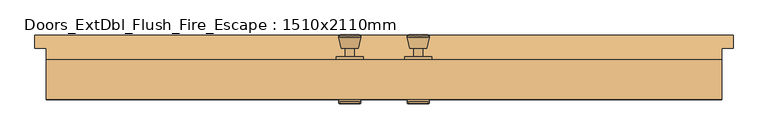
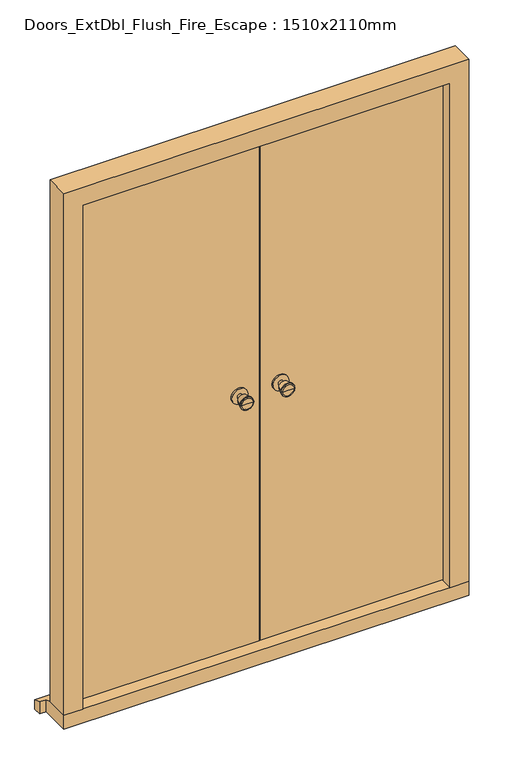
"""IFC4 building model written with IfcOpenShell, lengths in millimetres: door geometry, Doors_ExtDbl_Flush_Fire_Escape : 1510x2110mm."""

import ifcopenshell
import ifcopenshell.guid

model = None  # the IFC model being written
_history = None  # IfcOwnerHistory: only IFC2X3 demands one
_inside = {}  # id of a spatial element -> (the spatial element, [elements in it])
_under = {}  # id of a project, library or spatial element -> (it, [spatial elements below it])
_declared = {}  # id of a project -> (the project, [libraries it declares])
_typed = {}  # id of a type object -> (the type object, [elements of that type])
_made_of = {}  # id of a material, layer set ... -> (it, [elements and type objects made of it])


def new_model(schema):
    """Start an empty IFC model of exactly this schema.

    Asked for "IFC4X3", IfcOpenShell would pick the latest addendum, in which some entities
    have other attributes; the version numbers below select the first issue.
    IFC2X3 requires an IfcOwnerHistory on every rooted entity: one is made here for all.
    """
    global model, _history
    if schema == "IFC4X3":
        model = ifcopenshell.file(schema_version=(4, 3, 0, 0))
    else:
        model = ifcopenshell.file(schema=schema)
    _inside.clear()
    _under.clear()
    _declared.clear()
    _typed.clear()
    _made_of.clear()
    _history = None
    if model.schema == "IFC2X3":
        org = make("IfcOrganization", Name="unknown")
        user = make(
            "IfcPersonAndOrganization",
            ThePerson=make("IfcPerson", FamilyName="unknown"),
            TheOrganization=org,
        )
        app = make(
            "IfcApplication",
            ApplicationDeveloper=org,
            Version="unknown",
            ApplicationFullName="unknown",
            ApplicationIdentifier="unknown",
        )
        _history = make(
            "IfcOwnerHistory",
            OwningUser=user,
            OwningApplication=app,
            ChangeAction="ADDED",
            CreationDate=0,
        )
    return model


def make(cls, **values):
    """One entity of the class cls with the attributes given. An attribute that is None is left unset."""
    return model.create_entity(
        cls, **{name: value for name, value in values.items() if value is not None}
    )


def rooted(cls, **values):
    """An entity with a GlobalId (a new one), such as an element, a storey or a relation."""
    return make(cls, GlobalId=ifcopenshell.guid.new(), OwnerHistory=_history, **values)


def si_unit(unit_type, name, prefix=None):
    """IfcSIUnit, for example si_unit("LENGTHUNIT", "METRE", prefix="MILLI")."""
    return make("IfcSIUnit", UnitType=unit_type, Prefix=prefix, Name=name)


def assignment(units):
    """IfcUnitAssignment: the units of a project."""
    return None if units is None else make("IfcUnitAssignment", Units=units)


def point(xyz):
    """IfcCartesianPoint."""
    return None if xyz is None else make("IfcCartesianPoint", Coordinates=xyz)


def direction(xyz):
    """IfcDirection."""
    return None if xyz is None else make("IfcDirection", DirectionRatios=xyz)


def frame(location, z_axis=None, x_axis=None):
    """IfcAxis2Placement3D, a coordinate frame: its origin and axes. An axis left out is left unset."""
    return make(
        "IfcAxis2Placement3D",
        Location=point(location),
        Axis=direction(z_axis),
        RefDirection=direction(x_axis),
    )


def frame_2d(location, x_axis=None):
    """IfcAxis2Placement2D, a coordinate frame in the plane: its origin and x axis."""
    return make(
        "IfcAxis2Placement2D", Location=point(location), RefDirection=direction(x_axis)
    )


def origin():
    """The frame at (0, 0, 0) with its axes left unset."""
    return frame((0.0, 0.0, 0.0))


def place(relative_to, where):
    """IfcLocalPlacement: puts the frame where relative to a parent placement (None: the world)."""
    return make(
        "IfcLocalPlacement", PlacementRelTo=relative_to, RelativePlacement=where
    )


def context(
    kind, dimensions, precision=None, world=None, true_north=None, identifier=None
):
    """IfcGeometricRepresentationContext, for example the 3D "Model" context."""
    return make(
        "IfcGeometricRepresentationContext",
        ContextIdentifier=identifier,
        ContextType=kind,
        CoordinateSpaceDimension=dimensions,
        Precision=precision,
        WorldCoordinateSystem=world,
        TrueNorth=true_north,
    )


def project(units=None, contexts=None):
    """IfcProject with its units and contexts."""
    return rooted(
        "IfcProject",
        Name="project",
        RepresentationContexts=contexts,
        UnitsInContext=assignment(units),
    )


def spatial(cls, under=None, at=None, **own):
    """A site, building, storey or space (cls), placed at a placement, below another one or the project."""
    s = rooted(cls, ObjectPlacement=at, **own)
    if under is not None:
        _under.setdefault(under.id(), (under, []))[1].append(s)
    return s


def polyline(points):
    """IfcPolyline through the points."""
    return make("IfcPolyline", Points=[point(p) for p in points])


def circle_curve(where, radius):
    """IfcCircle in the frame where."""
    return make("IfcCircle", Position=where, Radius=radius)


def trimmed(basis, trim1, trim2, sense, master):
    """IfcTrimmedCurve: the piece of a basis curve between two trims."""
    return make(
        "IfcTrimmedCurve",
        BasisCurve=basis,
        Trim1=trim1,
        Trim2=trim2,
        SenseAgreement=sense,
        MasterRepresentation=master,
    )


def segment(curve, same_sense, transition):
    """IfcCompositeCurveSegment."""
    return make(
        "IfcCompositeCurveSegment",
        Transition=transition,
        SameSense=same_sense,
        ParentCurve=curve,
    )


def composite_curve(segments, self_intersect=None):
    """IfcCompositeCurve: segments joined end to end."""
    return make("IfcCompositeCurve", Segments=segments, SelfIntersect=self_intersect)


def outline(outer, holes=None, kind="AREA"):
    """IfcArbitraryClosedProfileDef: a profile drawn as a closed curve; with holes, ...WithVoids."""
    if holes is None:
        return make("IfcArbitraryClosedProfileDef", ProfileType=kind, OuterCurve=outer)
    return make(
        "IfcArbitraryProfileDefWithVoids",
        ProfileType=kind,
        OuterCurve=outer,
        InnerCurves=holes,
    )


def extrude(swept, where, along, depth):
    """IfcExtrudedAreaSolid: the profile swept, set in the frame where, extruded along a direction by depth."""
    return make(
        "IfcExtrudedAreaSolid",
        SweptArea=swept,
        Position=where,
        ExtrudedDirection=direction(along),
        Depth=depth,
    )


def faces_of(points, faces, orient=None, outer=None):
    """IfcFace entities. A face is a list of loops; a loop is a list of indices into points, from 0.

    orient and outer hold one flag for each loop. By default every Orientation is true, the
    first loop of a face is its IfcFaceOuterBound and the others are IfcFaceBound.
    """
    made = []
    for i, loops in enumerate(faces):
        bounds = []
        for j, loop in enumerate(loops):
            is_outer = j == 0 if outer is None else outer[i][j]
            bounds.append(
                make(
                    "IfcFaceOuterBound" if is_outer else "IfcFaceBound",
                    Bound=make("IfcPolyLoop", Polygon=[points[k] for k in loop]),
                    Orientation=True if orient is None else orient[i][j],
                )
            )
        made.append(make("IfcFace", Bounds=bounds))
    return made


def faceted_brep(points, faces, orient=None, outer=None, voids=None):
    """IfcFacetedBrep: a solid bounded by flat faces; with voids (closed shells), ...WithVoids."""
    shared = [point(p) for p in points]
    hull = make("IfcClosedShell", CfsFaces=faces_of(shared, faces, orient, outer))
    if voids is None:
        return make("IfcFacetedBrep", Outer=hull)
    return make(
        "IfcFacetedBrepWithVoids",
        Outer=hull,
        Voids=[
            make(cls, CfsFaces=faces_of(shared, fs, o, b)) for cls, fs, o, b in voids
        ],
    )


def shape(context_of_items, identifier, shape_type, items):
    """IfcShapeRepresentation: the items that make up one representation, for example the "Body"."""
    return make(
        "IfcShapeRepresentation",
        ContextOfItems=context_of_items,
        RepresentationIdentifier=identifier,
        RepresentationType=shape_type,
        Items=items,
    )


def source(mapping_origin, context_of_items, identifier, shape_type, items):
    """IfcRepresentationMap: a shape defined once, which mapped items show again and again."""
    return make(
        "IfcRepresentationMap",
        MappingOrigin=mapping_origin,
        MappedRepresentation=shape(context_of_items, identifier, shape_type, items),
    )


def transform(
    local_origin,
    x_axis=None,
    y_axis=None,
    z_axis=None,
    scale=None,
    scale2=None,
    scale3=None,
    uniform=True,
):
    """IfcCartesianTransformationOperator3D, or its non-uniform kind. x_axis, y_axis, z_axis: its Axis1, 2, 3."""
    if uniform:
        return make(
            "IfcCartesianTransformationOperator3D",
            Axis1=direction(x_axis),
            Axis2=direction(y_axis),
            LocalOrigin=point(local_origin),
            Scale=scale,
            Axis3=direction(z_axis),
        )
    return make(
        "IfcCartesianTransformationOperator3DnonUniform",
        Axis1=direction(x_axis),
        Axis2=direction(y_axis),
        LocalOrigin=point(local_origin),
        Scale=scale,
        Axis3=direction(z_axis),
        Scale2=scale2,
        Scale3=scale3,
    )


def mapped(mapping_source, mapping_target):
    """IfcMappedItem: shows the shape of a source again, moved by a transform."""
    return make(
        "IfcMappedItem", MappingSource=mapping_source, MappingTarget=mapping_target
    )


def made_of(thing, what):
    """Note that an element or type object is made of a material, layer set ...; save() writes the relation."""
    if what is not None:
        _made_of.setdefault(what.id(), (what, []))[1].append(thing)
    return thing


def element(
    cls,
    number,
    at=None,
    inside=None,
    cuts=None,
    type_object=None,
    material=None,
    context=None,
    identifier="Body",
    shape_type=None,
    held_by="IfcProductDefinitionShape",
    body=None,
    shapes=None,
    **own,
):
    """One element of the class cls, such as IfcWall. Its Tag is "e" and its number.

    at: its placement. inside: the storey or other place that contains it. cuts: it is an
    opening in that element (IfcRelVoidsElement). A single representation is given by context,
    identifier, shape_type and body (its items); several are given by shapes. held_by: the class
    of the entity that holds the representations. save() writes the other relations.
    """
    e = rooted(cls, Tag="e%d" % number, ObjectPlacement=at, **own)
    if body is not None:
        shapes = [shape(context, identifier, shape_type, body)]
    if shapes is not None:
        e.Representation = make(held_by, Representations=shapes)
    if inside is not None:
        _inside.setdefault(inside.id(), (inside, []))[1].append(e)
    if cuts is not None:
        rooted(
            "IfcRelVoidsElement", RelatingBuildingElement=cuts, RelatedOpeningElement=e
        )
    if type_object is not None:
        _typed.setdefault(type_object.id(), (type_object, []))[1].append(e)
    return made_of(e, material)


def aggregate(whole, parts):
    """IfcRelAggregates: a whole, such as a stair, and the parts it consists of."""
    return rooted("IfcRelAggregates", RelatingObject=whole, RelatedObjects=parts)


def save(model, path):
    """Write the relations noted so far, then the file.

    IfcRelAggregates (storeys below a building ...), IfcRelContainedInSpatialStructure (elements
    in a storey), IfcRelDefinesByType, IfcRelAssociatesMaterial and IfcRelDeclares: one each for
    every whole, place, type object, material and project.
    """
    for whole, parts in _under.values():
        aggregate(whole, parts)
    for where, things in _inside.values():
        rooted(
            "IfcRelContainedInSpatialStructure",
            RelatedElements=things,
            RelatingStructure=where,
        )
    for kind, things in _typed.values():
        rooted("IfcRelDefinesByType", RelatedObjects=things, RelatingType=kind)
    for what, things in _made_of.values():
        rooted("IfcRelAssociatesMaterial", RelatedObjects=things, RelatingMaterial=what)
    for by, libraries in _declared.values():
        rooted("IfcRelDeclares", RelatingContext=by, RelatedDefinitions=libraries)
    model.write(path)


def plane_surface(at):
    """IfcPlane: the flat surface through the origin of the frame at, square to its z axis."""
    return make("IfcPlane", Position=at)


def cylinder_surface(at, radius):
    """IfcCylindricalSurface: all points at the distance radius from the z axis of the frame at."""
    return make("IfcCylindricalSurface", Position=at, Radius=radius)


def revolved_surface(curve, axis_point, axis_direction):
    """IfcSurfaceOfRevolution: the curve turned about the line through axis_point along axis_direction."""
    return make(
        "IfcSurfaceOfRevolution",
        SweptCurve=make("IfcArbitraryOpenProfileDef", ProfileType="CURVE", Curve=curve),
        AxisPosition=make("IfcAxis1Placement", Location=point(axis_point), Axis=direction(axis_direction)),
    )


def advanced_brep(points, edges, surfaces, faces):
    """IfcAdvancedBrep: a solid bounded by faces that lie on surfaces and meet in shared edges.

    An edge is (start, end): straight between two places in points (the first is 0);
    or (start, end, curve); or (start, end, curve, False) where it runs against its curve.
    A face is (place in surfaces, loops), or (place, loops, False) where it looks against
    its surface's normal. A loop lists edges by number (the first is 1), with a minus sign
    where the edge is run from its end to its start. The first loop is the outer one.
    """
    corners = [point(p) for p in points]
    vertices = [make("IfcVertexPoint", VertexGeometry=c) for c in corners]
    made = []
    for start, end, *more in edges:
        made.append(
            make(
                "IfcEdgeCurve",
                EdgeStart=vertices[start],
                EdgeEnd=vertices[end],
                EdgeGeometry=more[0] if more else make("IfcPolyline", Points=[corners[start], corners[end]]),
                SameSense=more[1] if len(more) > 1 else True,
            )
        )
    hull = []
    for where, loops, *sense in faces:
        bounds = []
        for j, loop in enumerate(loops):
            ring = [make("IfcOrientedEdge", EdgeElement=made[abs(k) - 1], Orientation=k > 0) for k in loop]
            bounds.append(
                make(
                    "IfcFaceOuterBound" if j == 0 else "IfcFaceBound",
                    Bound=make("IfcEdgeLoop", EdgeList=ring),
                    Orientation=True,
                )
            )
        hull.append(make("IfcAdvancedFace", Bounds=bounds, FaceSurface=surfaces[where], SameSense=sense[0] if sense else True))
    return make("IfcAdvancedBrep", Outer=make("IfcClosedShell", CfsFaces=hull))


def doors_extdbl_flush_fire_escape_1510x2110mm_f48bbf68(model_context):
    return source(origin(), model_context, "Body", "SolidModel", [
        advanced_brep(
        [(-76.5, 156.0, 1050.0), (-86.5, 156.0, 1050.0), (-66.5, 156.0, 1050.0), (-96.9758676, 205.0, 1050.0), (-76.5, 205.0, 1050.0), (-56.0241324, 205.0, 1050.0), (-101.5, 203.1721319, 1050.0), (-51.5, 203.1721319, 1050.0), (-101.5, 199.7084537, 1050.0), (-51.5, 199.7084537, 1050.0), (-95.136236, 175.0, 1050.0), (-57.863764, 175.0, 1050.0), (-86.5, 175.0, 1050.0), (-66.5, 175.0, 1050.0)],
        [
            (0, 1),
            (1, 2, circle_curve(frame((-76.5, 156.0, 1050.0), z_axis=(0.0, -1.0, 0.0), x_axis=(1.0, 0.0, 0.0)), 10.0)),
            (2, 0),
            (2, 1, circle_curve(frame((-76.5, 156.0, 1050.0), z_axis=(0.0, -1.0, 0.0), x_axis=(1.0, 0.0, 0.0)), 10.0)),
            (3, 4),
            (4, 5),
            (5, 3, circle_curve(frame((-76.5, 205.0, 1050.0), z_axis=(0.0, 1.0, 0.0), x_axis=(1.0, 0.0, 0.0)), 20.4758676)),
            (3, 5, circle_curve(frame((-76.5, 205.0, 1050.0), z_axis=(0.0, 1.0, 0.0), x_axis=(1.0, 0.0, 0.0)), 20.4758676)),
            (6, 3),
            (5, 7),
            (7, 6, circle_curve(frame((-76.5, 203.1721319, 1050.0), z_axis=(0.0, 1.0, 0.0), x_axis=(1.0, 0.0, 0.0)), 25.0)),
            (6, 7, circle_curve(frame((-76.5, 203.1721319, 1050.0), z_axis=(0.0, 1.0, 0.0), x_axis=(1.0, 0.0, 0.0)), 25.0)),
            (8, 6),
            (7, 9),
            (9, 8, circle_curve(frame((-76.5, 199.7084537, 1050.0), z_axis=(0.0, 1.0, 0.0), x_axis=(1.0, 0.0, 0.0)), 25.0)),
            (8, 9, circle_curve(frame((-76.5, 199.7084537, 1050.0), z_axis=(0.0, 1.0, 0.0), x_axis=(1.0, 0.0, 0.0)), 25.0)),
            (10, 8),
            (9, 11),
            (11, 10, circle_curve(frame((-76.5, 175.0, 1050.0), z_axis=(0.0, 1.0, 0.0), x_axis=(1.0, 0.0, 0.0)), 18.636236)),
            (10, 11, circle_curve(frame((-76.5, 175.0, 1050.0), z_axis=(0.0, 1.0, 0.0), x_axis=(1.0, 0.0, 0.0)), 18.636236)),
            (12, 10),
            (11, 13),
            (13, 12, circle_curve(frame((-76.5, 175.0, 1050.0), z_axis=(0.0, 1.0, 0.0), x_axis=(1.0, 0.0, 0.0)), 10.0)),
            (12, 13, circle_curve(frame((-76.5, 175.0, 1050.0), z_axis=(0.0, 1.0, 0.0), x_axis=(1.0, 0.0, 0.0)), 10.0)),
            (1, 12),
            (13, 2),
        ],
        [
            plane_surface(frame((-76.5, 156.0, 1050.0), z_axis=(0.0, -1.0, 0.0), x_axis=(1.0, 0.0, 0.0))),
            plane_surface(frame((-76.5, 205.0, 1050.0), z_axis=(0.0, 1.0, 0.0), x_axis=(1.0, 0.0, 0.0))),
            revolved_surface(polyline([(-56.0241324, 205.0, 1050.0), (-51.5, 203.1721319, 1050.0)]), (-76.5, 156.0, 1050.0), (0.0, -1.0, 0.0)),
            cylinder_surface(frame((-76.5, 156.0, 1050.0), z_axis=(0.0, -1.0, 0.0), x_axis=(1.0, 0.0, 0.0)), 25.0),
            revolved_surface(polyline([(-51.5, 199.7084537, 1050.0), (-57.863764, 175.0, 1050.0)]), (-76.5, 156.0, 1050.0), (0.0, -1.0, 0.0)),
            plane_surface(frame((-76.5, 175.0, 1050.0), z_axis=(0.0, -1.0, 0.0), x_axis=(1.0, 0.0, 0.0))),
            cylinder_surface(frame((-76.5, 156.0, 1050.0), z_axis=(0.0, -1.0, 0.0), x_axis=(1.0, 0.0, 0.0)), 10.0),
        ],
        [
            (0, [[1, 2, 3]]),
            (0, [[-3, 4, -1]]),
            (1, [[5, 6, 7]]),
            (1, [[-6, -5, 8]]),
            (2, [[9, -7, 10, 11]]),
            (2, [[-10, -8, -9, 12]]),
            (3, [[13, -11, 14, 15]]),
            (3, [[-14, -12, -13, 16]]),
            (4, [[17, -15, 18, 19]]),
            (4, [[-18, -16, -17, 20]]),
            (5, [[21, -19, 22, 23]]),
            (5, [[-22, -20, -21, 24]]),
            (6, [[25, -23, 26, -2]]),
            (6, [[-26, -24, -25, -4]]),
        ],
    ),
        extrude(outline(composite_curve([segment(trimmed(circle_curve(frame_2d((1050.0, -76.5)), 30.0), [point((1050.0, -46.5))], [point((1050.0, -106.5))], False, "CARTESIAN"), True, "CONTINUOUS"), segment(trimmed(circle_curve(frame_2d((1050.0, -76.5)), 30.0), [point((1050.0, -106.5))], [point((1050.0, -46.5))], False, "CARTESIAN"), True, "CONTINUOUS")], self_intersect=False)), frame((0.0, 150.0, 0.0), z_axis=(0.0, 1.0, 0.0), x_axis=(0.0, 0.0, 1.0)), (0.0, 0.0, 1.0), 6.0),
        advanced_brep(
        [(-76.5, 100.0, 1050.0), (-66.5, 100.0, 1050.0), (-86.5, 100.0, 1050.0), (-96.9758676, 51.0, 1050.0), (-56.0241324, 51.0, 1050.0), (-76.5, 51.0, 1050.0), (-101.5, 52.8278681, 1050.0), (-51.5, 52.8278681, 1050.0), (-101.5, 56.2915463, 1050.0), (-51.5, 56.2915463, 1050.0), (-95.136236, 81.0, 1050.0), (-57.863764, 81.0, 1050.0), (-86.5, 81.0, 1050.0), (-66.5, 81.0, 1050.0)],
        [
            (0, 1),
            (1, 2, circle_curve(frame((-76.5, 100.0, 1050.0), z_axis=(0.0, 1.0, 0.0), x_axis=(1.0, 0.0, 0.0)), 10.0)),
            (2, 0),
            (2, 1, circle_curve(frame((-76.5, 100.0, 1050.0), z_axis=(0.0, 1.0, 0.0), x_axis=(1.0, 0.0, 0.0)), 10.0)),
            (3, 4, circle_curve(frame((-76.5, 51.0, 1050.0), z_axis=(0.0, -1.0, 0.0), x_axis=(1.0, 0.0, 0.0)), 20.4758676)),
            (4, 5),
            (5, 3),
            (4, 3, circle_curve(frame((-76.5, 51.0, 1050.0), z_axis=(0.0, -1.0, 0.0), x_axis=(1.0, 0.0, 0.0)), 20.4758676)),
            (6, 7, circle_curve(frame((-76.5, 52.8278681, 1050.0), z_axis=(0.0, -1.0, 0.0), x_axis=(1.0, 0.0, 0.0)), 25.0)),
            (7, 4),
            (3, 6),
            (7, 6, circle_curve(frame((-76.5, 52.8278681, 1050.0), z_axis=(0.0, -1.0, 0.0), x_axis=(1.0, 0.0, 0.0)), 25.0)),
            (8, 9, circle_curve(frame((-76.5, 56.2915463, 1050.0), z_axis=(0.0, -1.0, 0.0), x_axis=(1.0, 0.0, 0.0)), 25.0)),
            (9, 7),
            (6, 8),
            (9, 8, circle_curve(frame((-76.5, 56.2915463, 1050.0), z_axis=(0.0, -1.0, 0.0), x_axis=(1.0, 0.0, 0.0)), 25.0)),
            (10, 11, circle_curve(frame((-76.5, 81.0, 1050.0), z_axis=(0.0, -1.0, 0.0), x_axis=(1.0, 0.0, 0.0)), 18.636236)),
            (11, 9),
            (8, 10),
            (11, 10, circle_curve(frame((-76.5, 81.0, 1050.0), z_axis=(0.0, -1.0, 0.0), x_axis=(1.0, 0.0, 0.0)), 18.636236)),
            (12, 13, circle_curve(frame((-76.5, 81.0, 1050.0), z_axis=(0.0, -1.0, 0.0), x_axis=(1.0, 0.0, 0.0)), 10.0)),
            (13, 11),
            (10, 12),
            (13, 12, circle_curve(frame((-76.5, 81.0, 1050.0), z_axis=(0.0, -1.0, 0.0), x_axis=(1.0, 0.0, 0.0)), 10.0)),
            (1, 13),
            (12, 2),
        ],
        [
            plane_surface(frame((-76.5, 100.0, 1050.0), z_axis=(0.0, 1.0, 0.0), x_axis=(1.0, 0.0, 0.0))),
            plane_surface(frame((-76.5, 51.0, 1050.0), z_axis=(0.0, -1.0, 0.0), x_axis=(1.0, 0.0, 0.0))),
            revolved_surface(polyline([(-56.0241324, 51.0, 1050.0), (-51.5, 52.8278681, 1050.0)]), (-76.5, 100.0, 1050.0), (0.0, 1.0, 0.0)),
            cylinder_surface(frame((-76.5, 100.0, 1050.0), z_axis=(0.0, 1.0, 0.0), x_axis=(1.0, 0.0, 0.0)), 25.0),
            revolved_surface(polyline([(-51.5, 56.2915463, 1050.0), (-57.863764, 81.0, 1050.0)]), (-76.5, 100.0, 1050.0), (0.0, 1.0, 0.0)),
            plane_surface(frame((-76.5, 81.0, 1050.0), z_axis=(0.0, 1.0, 0.0), x_axis=(1.0, 0.0, 0.0))),
            cylinder_surface(frame((-76.5, 100.0, 1050.0), z_axis=(0.0, 1.0, 0.0), x_axis=(1.0, 0.0, 0.0)), 10.0),
        ],
        [
            (0, [[1, 2, 3]]),
            (0, [[-3, 4, -1]]),
            (1, [[5, 6, 7]]),
            (1, [[8, -7, -6]]),
            (2, [[9, 10, -5, 11]]),
            (2, [[12, -11, -8, -10]]),
            (3, [[13, 14, -9, 15]]),
            (3, [[16, -15, -12, -14]]),
            (4, [[17, 18, -13, 19]]),
            (4, [[20, -19, -16, -18]]),
            (5, [[21, 22, -17, 23]]),
            (5, [[24, -23, -20, -22]]),
            (6, [[-2, 25, -21, 26]]),
            (6, [[-4, -26, -24, -25]]),
        ],
    ),
        extrude(outline(composite_curve([segment(trimmed(circle_curve(frame_2d((1050.0, -76.5)), 30.0), [point((1050.0, -46.5))], [point((1050.0, -106.5))], False, "CARTESIAN"), True, "CONTINUOUS"), segment(trimmed(circle_curve(frame_2d((1050.0, -76.5)), 30.0), [point((1050.0, -106.5))], [point((1050.0, -46.5))], False, "CARTESIAN"), True, "CONTINUOUS")], self_intersect=False)), frame((0.0, 100.0, 0.0), z_axis=(0.0, 1.0, 0.0), x_axis=(0.0, 0.0, 1.0)), (0.0, 0.0, 1.0), 6.0),
        advanced_brep(
        [(76.5, 156.0, 1050.0), (66.5, 156.0, 1050.0), (86.5, 156.0, 1050.0), (96.9758676, 205.0, 1050.0), (56.0241324, 205.0, 1050.0), (76.5, 205.0, 1050.0), (101.5, 203.1721319, 1050.0), (51.5, 203.1721319, 1050.0), (101.5, 199.7084537, 1050.0), (51.5, 199.7084537, 1050.0), (95.136236, 175.0, 1050.0), (57.863764, 175.0, 1050.0), (86.5, 175.0, 1050.0), (66.5, 175.0, 1050.0)],
        [
            (0, 1),
            (1, 2, circle_curve(frame((76.5, 156.0, 1050.0), z_axis=(0.0, -1.0, 0.0), x_axis=(-1.0, 0.0, 0.0)), 10.0)),
            (2, 0),
            (2, 1, circle_curve(frame((76.5, 156.0, 1050.0), z_axis=(0.0, -1.0, 0.0), x_axis=(-1.0, 0.0, 0.0)), 10.0)),
            (3, 4, circle_curve(frame((76.5, 205.0, 1050.0), z_axis=(0.0, 1.0, 0.0), x_axis=(-1.0, 0.0, 0.0)), 20.4758676)),
            (4, 5),
            (5, 3),
            (4, 3, circle_curve(frame((76.5, 205.0, 1050.0), z_axis=(0.0, 1.0, 0.0), x_axis=(-1.0, 0.0, 0.0)), 20.4758676)),
            (6, 7, circle_curve(frame((76.5, 203.1721319, 1050.0), z_axis=(0.0, 1.0, 0.0), x_axis=(-1.0, 0.0, 0.0)), 25.0)),
            (7, 4),
            (3, 6),
            (7, 6, circle_curve(frame((76.5, 203.1721319, 1050.0), z_axis=(0.0, 1.0, 0.0), x_axis=(-1.0, 0.0, 0.0)), 25.0)),
            (8, 9, circle_curve(frame((76.5, 199.7084537, 1050.0), z_axis=(0.0, 1.0, 0.0), x_axis=(-1.0, 0.0, 0.0)), 25.0)),
            (9, 7),
            (6, 8),
            (9, 8, circle_curve(frame((76.5, 199.7084537, 1050.0), z_axis=(0.0, 1.0, 0.0), x_axis=(-1.0, 0.0, 0.0)), 25.0)),
            (10, 11, circle_curve(frame((76.5, 175.0, 1050.0), z_axis=(0.0, 1.0, 0.0), x_axis=(-1.0, 0.0, 0.0)), 18.636236)),
            (11, 9),
            (8, 10),
            (11, 10, circle_curve(frame((76.5, 175.0, 1050.0), z_axis=(0.0, 1.0, 0.0), x_axis=(-1.0, 0.0, 0.0)), 18.636236)),
            (12, 13, circle_curve(frame((76.5, 175.0, 1050.0), z_axis=(0.0, 1.0, 0.0), x_axis=(-1.0, 0.0, 0.0)), 10.0)),
            (13, 11),
            (10, 12),
            (13, 12, circle_curve(frame((76.5, 175.0, 1050.0), z_axis=(0.0, 1.0, 0.0), x_axis=(-1.0, 0.0, 0.0)), 10.0)),
            (1, 13),
            (12, 2),
        ],
        [
            plane_surface(frame((76.5, 156.0, 1050.0), z_axis=(0.0, -1.0, 0.0), x_axis=(-1.0, 0.0, 0.0))),
            plane_surface(frame((76.5, 205.0, 1050.0), z_axis=(0.0, 1.0, 0.0), x_axis=(-1.0, 0.0, 0.0))),
            revolved_surface(polyline([(56.0241324, 205.0, 1050.0), (51.5, 203.1721319, 1050.0)]), (76.5, 156.0, 1050.0), (0.0, -1.0, 0.0)),
            cylinder_surface(frame((76.5, 156.0, 1050.0), z_axis=(0.0, -1.0, 0.0), x_axis=(-1.0, 0.0, 0.0)), 25.0),
            revolved_surface(polyline([(51.5, 199.7084537, 1050.0), (57.863764, 175.0, 1050.0)]), (76.5, 156.0, 1050.0), (0.0, -1.0, 0.0)),
            plane_surface(frame((76.5, 175.0, 1050.0), z_axis=(0.0, -1.0, 0.0), x_axis=(-1.0, 0.0, 0.0))),
            cylinder_surface(frame((76.5, 156.0, 1050.0), z_axis=(0.0, -1.0, 0.0), x_axis=(-1.0, 0.0, 0.0)), 10.0),
        ],
        [
            (0, [[1, 2, 3]]),
            (0, [[-3, 4, -1]]),
            (1, [[5, 6, 7]]),
            (1, [[8, -7, -6]]),
            (2, [[9, 10, -5, 11]]),
            (2, [[12, -11, -8, -10]]),
            (3, [[13, 14, -9, 15]]),
            (3, [[16, -15, -12, -14]]),
            (4, [[17, 18, -13, 19]]),
            (4, [[20, -19, -16, -18]]),
            (5, [[21, 22, -17, 23]]),
            (5, [[24, -23, -20, -22]]),
            (6, [[-2, 25, -21, 26]]),
            (6, [[-4, -26, -24, -25]]),
        ],
    ),
        extrude(outline(composite_curve([segment(trimmed(circle_curve(frame_2d((1050.0, 76.5)), 30.0), [point((1050.0, 46.5))], [point((1050.0, 106.5))], False, "CARTESIAN"), True, "CONTINUOUS"), segment(trimmed(circle_curve(frame_2d((1050.0, 76.5)), 30.0), [point((1050.0, 106.5))], [point((1050.0, 46.5))], False, "CARTESIAN"), True, "CONTINUOUS")], self_intersect=False)), frame((0.0, 150.0, 0.0), z_axis=(0.0, 1.0, 0.0), x_axis=(0.0, 0.0, 1.0)), (0.0, 0.0, 1.0), 6.0),
        advanced_brep(
        [(76.5, 100.0, 1050.0), (86.5, 100.0, 1050.0), (66.5, 100.0, 1050.0), (96.9758676, 51.0, 1050.0), (76.5, 51.0, 1050.0), (56.0241324, 51.0, 1050.0), (101.5, 52.8278681, 1050.0), (51.5, 52.8278681, 1050.0), (101.5, 56.2915463, 1050.0), (51.5, 56.2915463, 1050.0), (95.136236, 81.0, 1050.0), (57.863764, 81.0, 1050.0), (86.5, 81.0, 1050.0), (66.5, 81.0, 1050.0)],
        [
            (0, 1),
            (1, 2, circle_curve(frame((76.5, 100.0, 1050.0), z_axis=(0.0, 1.0, 0.0), x_axis=(-1.0, 0.0, 0.0)), 10.0)),
            (2, 0),
            (2, 1, circle_curve(frame((76.5, 100.0, 1050.0), z_axis=(0.0, 1.0, 0.0), x_axis=(-1.0, 0.0, 0.0)), 10.0)),
            (3, 4),
            (4, 5),
            (5, 3, circle_curve(frame((76.5, 51.0, 1050.0), z_axis=(0.0, -1.0, 0.0), x_axis=(-1.0, 0.0, 0.0)), 20.4758676)),
            (3, 5, circle_curve(frame((76.5, 51.0, 1050.0), z_axis=(0.0, -1.0, 0.0), x_axis=(-1.0, 0.0, 0.0)), 20.4758676)),
            (6, 3),
            (5, 7),
            (7, 6, circle_curve(frame((76.5, 52.8278681, 1050.0), z_axis=(0.0, -1.0, 0.0), x_axis=(-1.0, 0.0, 0.0)), 25.0)),
            (6, 7, circle_curve(frame((76.5, 52.8278681, 1050.0), z_axis=(0.0, -1.0, 0.0), x_axis=(-1.0, 0.0, 0.0)), 25.0)),
            (8, 6),
            (7, 9),
            (9, 8, circle_curve(frame((76.5, 56.2915463, 1050.0), z_axis=(0.0, -1.0, 0.0), x_axis=(-1.0, 0.0, 0.0)), 25.0)),
            (8, 9, circle_curve(frame((76.5, 56.2915463, 1050.0), z_axis=(0.0, -1.0, 0.0), x_axis=(-1.0, 0.0, 0.0)), 25.0)),
            (10, 8),
            (9, 11),
            (11, 10, circle_curve(frame((76.5, 81.0, 1050.0), z_axis=(0.0, -1.0, 0.0), x_axis=(-1.0, 0.0, 0.0)), 18.636236)),
            (10, 11, circle_curve(frame((76.5, 81.0, 1050.0), z_axis=(0.0, -1.0, 0.0), x_axis=(-1.0, 0.0, 0.0)), 18.636236)),
            (12, 10),
            (11, 13),
            (13, 12, circle_curve(frame((76.5, 81.0, 1050.0), z_axis=(0.0, -1.0, 0.0), x_axis=(-1.0, 0.0, 0.0)), 10.0)),
            (12, 13, circle_curve(frame((76.5, 81.0, 1050.0), z_axis=(0.0, -1.0, 0.0), x_axis=(-1.0, 0.0, 0.0)), 10.0)),
            (1, 12),
            (13, 2),
        ],
        [
            plane_surface(frame((76.5, 100.0, 1050.0), z_axis=(0.0, 1.0, 0.0), x_axis=(-1.0, 0.0, 0.0))),
            plane_surface(frame((76.5, 51.0, 1050.0), z_axis=(0.0, -1.0, 0.0), x_axis=(-1.0, 0.0, 0.0))),
            revolved_surface(polyline([(56.0241324, 51.0, 1050.0), (51.5, 52.8278681, 1050.0)]), (76.5, 100.0, 1050.0), (0.0, 1.0, 0.0)),
            cylinder_surface(frame((76.5, 100.0, 1050.0), z_axis=(0.0, 1.0, 0.0), x_axis=(-1.0, 0.0, 0.0)), 25.0),
            revolved_surface(polyline([(51.5, 56.2915463, 1050.0), (57.863764, 81.0, 1050.0)]), (76.5, 100.0, 1050.0), (0.0, 1.0, 0.0)),
            plane_surface(frame((76.5, 81.0, 1050.0), z_axis=(0.0, 1.0, 0.0), x_axis=(-1.0, 0.0, 0.0))),
            cylinder_surface(frame((76.5, 100.0, 1050.0), z_axis=(0.0, 1.0, 0.0), x_axis=(-1.0, 0.0, 0.0)), 10.0),
        ],
        [
            (0, [[1, 2, 3]]),
            (0, [[-3, 4, -1]]),
            (1, [[5, 6, 7]]),
            (1, [[-6, -5, 8]]),
            (2, [[9, -7, 10, 11]]),
            (2, [[-10, -8, -9, 12]]),
            (3, [[13, -11, 14, 15]]),
            (3, [[-14, -12, -13, 16]]),
            (4, [[17, -15, 18, 19]]),
            (4, [[-18, -16, -17, 20]]),
            (5, [[21, -19, 22, 23]]),
            (5, [[-22, -20, -21, 24]]),
            (6, [[25, -23, 26, -2]]),
            (6, [[-26, -24, -25, -4]]),
        ],
    ),
        extrude(outline(composite_curve([segment(trimmed(circle_curve(frame_2d((1050.0, 76.5)), 30.0), [point((1050.0, 46.5))], [point((1050.0, 106.5))], False, "CARTESIAN"), True, "CONTINUOUS"), segment(trimmed(circle_curve(frame_2d((1050.0, 76.5)), 30.0), [point((1050.0, 106.5))], [point((1050.0, 46.5))], False, "CARTESIAN"), True, "CONTINUOUS")], self_intersect=False)), frame((0.0, 100.0, 0.0), z_axis=(0.0, 1.0, 0.0), x_axis=(0.0, 0.0, 1.0)), (0.0, 0.0, 1.0), 6.0),
        faceted_brep([(706.5, 150.0, 54.5), (755.0, 150.0, 54.5), (755.0, 61.0, 54.5), (684.5, 61.0, 54.5), (684.5, 103.0, 54.5), (706.5, 103.0, 54.5), (706.5, 150.0, 2061.5), (-706.5, 150.0, 2061.5), (-706.5, 150.0, 54.5), (-755.0, 150.0, 54.5), (-755.0, 150.0, 2110.0), (755.0, 150.0, 2110.0), (755.0, 61.0, 2110.0), (-755.0, 61.0, 2110.0), (-755.0, 61.0, 54.5), (-684.5, 61.0, 54.5), (-684.5, 61.0, 2039.5), (684.5, 61.0, 2039.5), (684.5, 103.0, 2039.5), (-684.5, 103.0, 2039.5), (-684.5, 103.0, 54.5), (-706.5, 103.0, 54.5), (-706.5, 103.0, 2061.5), (706.5, 103.0, 2061.5)], [[[0, 1, 2, 3, 4, 5]], [[1, 0, 6, 7, 8, 9, 10, 11]], [[2, 1, 11, 12]], [[3, 2, 12, 13, 14, 15, 16, 17]], [[4, 3, 17, 18]], [[5, 4, 18, 19, 20, 21, 22, 23]], [[0, 5, 23, 6]], [[7, 22, 21, 8]], [[8, 21, 20, 15, 14, 9]], [[13, 10, 9, 14]], [[19, 16, 15, 20]], [[12, 11, 10, 13]], [[18, 17, 16, 19]], [[6, 23, 22, 7]]]),
        extrude(outline(polyline([(1.5, 150.0), (703.5, 150.0), (703.5, 106.0), (1.5, 106.0), (1.5, 150.0)])), frame((0.0, 0.0, 58.5), z_axis=(0.0, 0.0, 1.0), x_axis=(1.0, 0.0, 0.0)), (0.0, 0.0, 1.0), 2000.0),
        extrude(outline(polyline([(-703.5, 150.0), (-1.5, 150.0), (-1.5, 106.0), (-703.5, 106.0), (-703.5, 150.0)])), frame((0.0, 0.0, 58.5), z_axis=(0.0, 0.0, 1.0), x_axis=(1.0, 0.0, 0.0)), (0.0, 0.0, 1.0), 2000.0),
        faceted_brep([(780.0, 205.0, 0.0), (780.0, 205.0, 38.5947221), (780.0, 175.0, 47.2703282), (780.0, 175.0, 0.0), (-780.0, 205.0, 38.5947221), (-780.0, 205.0, 0.0), (-780.0, 175.0, 0.0), (-780.0, 175.0, 47.2703282), (755.0, 175.0, 0.0), (755.0, 61.0, 0.0), (-755.0, 61.0, 0.0), (-755.0, 175.0, 0.0), (-755.0, 175.0, 47.2703282), (-755.0, 150.0, 54.5), (755.0, 150.0, 54.5), (755.0, 175.0, 47.2703282), (-755.0, 61.0, 54.5), (755.0, 61.0, 54.5)], [[[0, 1, 2, 3]], [[4, 5, 6, 7]], [[5, 0, 3, 8, 9, 10, 11, 6]], [[1, 0, 5, 4]], [[1, 4, 7, 12, 13, 14, 15, 2]], [[13, 16, 17, 14]], [[16, 10, 9, 17]], [[12, 11, 10, 16, 13]], [[11, 12, 7, 6]], [[8, 15, 14, 17, 9]], [[15, 8, 3, 2]]]),
    ])


if __name__ == "__main__":
    model = new_model("IFC4")
    model_context = context("Model", 3, world=origin())
    ifc_project = project(units=[si_unit("LENGTHUNIT", "METRE", prefix="MILLI")], contexts=[model_context])
    site = spatial("IfcSite", under=ifc_project)
    building = spatial("IfcBuilding", under=site)
    placement = place(None, origin())
    doors_extdbl_flush_fire_escape_1510x2110mm_shape = doors_extdbl_flush_fire_escape_1510x2110mm_f48bbf68(model_context)
    element("IfcDoor", 1, ObjectType="Doors_ExtDbl_Flush_Fire_Escape : 1510x2110mm", at=placement, inside=building, context=model_context, shape_type="MappedRepresentation", body=[
        mapped(doors_extdbl_flush_fire_escape_1510x2110mm_shape, transform((0.0, 0.0, 0.0), x_axis=(1.0, 0.0, 0.0), y_axis=(0.0, 1.0, 0.0), z_axis=(0.0, 0.0, 1.0))),
    ])
    save(model, "model.ifc")

# Revit data of these elements
# Type "Doors_ExtDbl_Flush_Fire_Escape : 1510x2110mm"
#   Type Mark = "50"
#   Type Comments = "External Double"
#   Operation = "DoubleDoorSingleSwing"
#   Construction Type Id = "MDOOR"
#   Keynote = "L20"
#   Description = "External Opening Double Doors"
#   Analytic Construction = "Metal"
#   Wrap Layers (Ext) from Ext = 102.5 mm
#   Wrap Layers (Int) from Ext = 177.5 mm
#   Thickness = 44 mm
#   Rough Width = 1510 mm
#   Rough Height = 2110 mm
#   O/A Frame Width = 64 mm
#   Heat Transfer Coefficient (U) = 3.7021 W/(m²·K)
#   Handle Z Distance = 1050 mm
#   FrameWidth = 42 mm
#   FrameOffset - External = 25 mm
#   FrameDepth = 89 mm
#   Door Panel Width = 702 mm
#   Door Panel Thickness = 44 mm
#   Door Panel Height = 2000 mm
#   Cill Thickness = 54.5 mm
#   Cill Projection = 30 mm
#   Handle X Distance = 75 mm
#   Height = 2110 mm
#   Structural Tolerance = 6.5 mm
#   Tolerance = 3 mm
#   Undercut = 4 mm
#   Width = 1510 mm
#   Cill Extension = 25 mm
#   Cavity Closer Width = 50 mm
#   Cavity Closer Offset from Ext = 102.5 mm
#   Cavity Closer Depth = 85 mm
#   Vis - Ironmongery = yes
#   Vis - Cavity Closers = yes
#   Define Thermal Properties by = 1
#   Function = 1
#   Material Door = Door - Panel
#   Material Frame = Door - Frame/Mullion
#   Material Ironmongery = Door - Handle
#   Visual Light Transmittance = 0
#   Solar Heat Gain Coefficient = 0
#   Wall Closure = (empty or 0)
# Element 1 (IfcDoor, "Doors_ExtDbl_Flush_Fire_Escape : 1510x2110mm")
#   Materials on its faces: "Door - Handle", "Door - Frame/Mullion", "Door - Panel"
# Materials
#   "Door - Panel": class "Wood", colour RGB 210 159 95, transparency 0, Keynote = "L20", Cost = 0
#   "Door - Frame/Mullion": class "Wood", colour RGB 212 179 113, transparency 0, Keynote = "L20", Cost = 0
#   "Door - Handle": class "Miscellaneous", colour RGB 0 0 0, transparency 0, Keynote = "P21", Cost = 0
